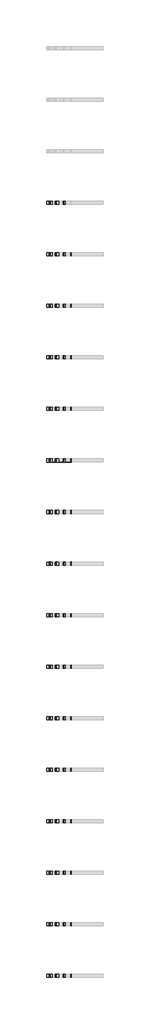
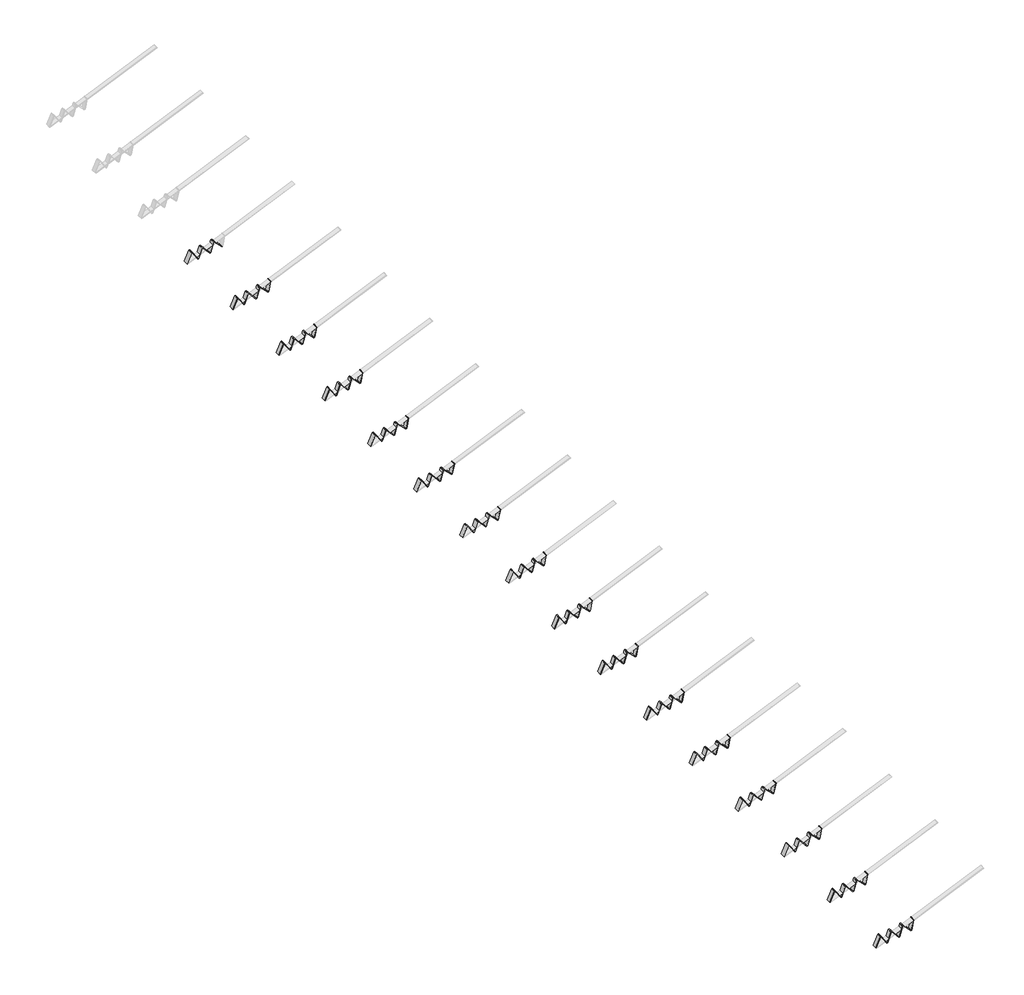
# One storey, part 1 of 4: 111 beams.
"""IFC4 building model written with IfcOpenShell, lengths in millimetres."""

import ifcopenshell
import ifcopenshell.guid

model = None  # the IFC model being written
_history = None  # IfcOwnerHistory: only IFC2X3 demands one
_inside = {}  # id of a spatial element -> (the spatial element, [elements in it])
_under = {}  # id of a project, library or spatial element -> (it, [spatial elements below it])
_declared = {}  # id of a project -> (the project, [libraries it declares])
_typed = {}  # id of a type object -> (the type object, [elements of that type])
_made_of = {}  # id of a material, layer set ... -> (it, [elements and type objects made of it])


def new_model(schema):
    """Start an empty IFC model of exactly this schema.

    Asked for "IFC4X3", IfcOpenShell would pick the latest addendum, in which some entities
    have other attributes; the version numbers below select the first issue.
    IFC2X3 requires an IfcOwnerHistory on every rooted entity: one is made here for all.
    """
    global model, _history
    if schema == "IFC4X3":
        model = ifcopenshell.file(schema_version=(4, 3, 0, 0))
    else:
        model = ifcopenshell.file(schema=schema)
    _inside.clear()
    _under.clear()
    _declared.clear()
    _typed.clear()
    _made_of.clear()
    _history = None
    if model.schema == "IFC2X3":
        org = make("IfcOrganization", Name="unknown")
        user = make(
            "IfcPersonAndOrganization",
            ThePerson=make("IfcPerson", FamilyName="unknown"),
            TheOrganization=org,
        )
        app = make(
            "IfcApplication",
            ApplicationDeveloper=org,
            Version="unknown",
            ApplicationFullName="unknown",
            ApplicationIdentifier="unknown",
        )
        _history = make(
            "IfcOwnerHistory",
            OwningUser=user,
            OwningApplication=app,
            ChangeAction="ADDED",
            CreationDate=0,
        )
    return model


def make(cls, **values):
    """One entity of the class cls with the attributes given. An attribute that is None is left unset."""
    return model.create_entity(
        cls, **{name: value for name, value in values.items() if value is not None}
    )


def rooted(cls, **values):
    """An entity with a GlobalId (a new one), such as an element, a storey or a relation."""
    return make(cls, GlobalId=ifcopenshell.guid.new(), OwnerHistory=_history, **values)


def si_unit(unit_type, name, prefix=None):
    """IfcSIUnit, for example si_unit("LENGTHUNIT", "METRE", prefix="MILLI")."""
    return make("IfcSIUnit", UnitType=unit_type, Prefix=prefix, Name=name)


def assignment(units):
    """IfcUnitAssignment: the units of a project."""
    return None if units is None else make("IfcUnitAssignment", Units=units)


def point(xyz):
    """IfcCartesianPoint."""
    return None if xyz is None else make("IfcCartesianPoint", Coordinates=xyz)


def direction(xyz):
    """IfcDirection."""
    return None if xyz is None else make("IfcDirection", DirectionRatios=xyz)


def frame(location, z_axis=None, x_axis=None):
    """IfcAxis2Placement3D, a coordinate frame: its origin and axes. An axis left out is left unset."""
    return make(
        "IfcAxis2Placement3D",
        Location=point(location),
        Axis=direction(z_axis),
        RefDirection=direction(x_axis),
    )


def origin():
    """The frame at (0, 0, 0) with its axes left unset."""
    return frame((0.0, 0.0, 0.0))


def place(relative_to, where):
    """IfcLocalPlacement: puts the frame where relative to a parent placement (None: the world)."""
    return make(
        "IfcLocalPlacement", PlacementRelTo=relative_to, RelativePlacement=where
    )


def context(
    kind, dimensions, precision=None, world=None, true_north=None, identifier=None
):
    """IfcGeometricRepresentationContext, for example the 3D "Model" context."""
    return make(
        "IfcGeometricRepresentationContext",
        ContextIdentifier=identifier,
        ContextType=kind,
        CoordinateSpaceDimension=dimensions,
        Precision=precision,
        WorldCoordinateSystem=world,
        TrueNorth=true_north,
    )


def project(units=None, contexts=None):
    """IfcProject with its units and contexts."""
    return rooted(
        "IfcProject",
        Name="project",
        RepresentationContexts=contexts,
        UnitsInContext=assignment(units),
    )


def spatial(cls, under=None, at=None, **own):
    """A site, building, storey or space (cls), placed at a placement, below another one or the project."""
    s = rooted(cls, ObjectPlacement=at, **own)
    if under is not None:
        _under.setdefault(under.id(), (under, []))[1].append(s)
    return s


def polyline(points):
    """IfcPolyline through the points."""
    return make("IfcPolyline", Points=[point(p) for p in points])


def outline(outer, holes=None, kind="AREA"):
    """IfcArbitraryClosedProfileDef: a profile drawn as a closed curve; with holes, ...WithVoids."""
    if holes is None:
        return make("IfcArbitraryClosedProfileDef", ProfileType=kind, OuterCurve=outer)
    return make(
        "IfcArbitraryProfileDefWithVoids",
        ProfileType=kind,
        OuterCurve=outer,
        InnerCurves=holes,
    )


def extrude(swept, where, along, depth):
    """IfcExtrudedAreaSolid: the profile swept, set in the frame where, extruded along a direction by depth."""
    return make(
        "IfcExtrudedAreaSolid",
        SweptArea=swept,
        Position=where,
        ExtrudedDirection=direction(along),
        Depth=depth,
    )


def shape(context_of_items, identifier, shape_type, items):
    """IfcShapeRepresentation: the items that make up one representation, for example the "Body"."""
    return make(
        "IfcShapeRepresentation",
        ContextOfItems=context_of_items,
        RepresentationIdentifier=identifier,
        RepresentationType=shape_type,
        Items=items,
    )


def source(mapping_origin, context_of_items, identifier, shape_type, items):
    """IfcRepresentationMap: a shape defined once, which mapped items show again and again."""
    return make(
        "IfcRepresentationMap",
        MappingOrigin=mapping_origin,
        MappedRepresentation=shape(context_of_items, identifier, shape_type, items),
    )


def transform(
    local_origin,
    x_axis=None,
    y_axis=None,
    z_axis=None,
    scale=None,
    scale2=None,
    scale3=None,
    uniform=True,
):
    """IfcCartesianTransformationOperator3D, or its non-uniform kind. x_axis, y_axis, z_axis: its Axis1, 2, 3."""
    if uniform:
        return make(
            "IfcCartesianTransformationOperator3D",
            Axis1=direction(x_axis),
            Axis2=direction(y_axis),
            LocalOrigin=point(local_origin),
            Scale=scale,
            Axis3=direction(z_axis),
        )
    return make(
        "IfcCartesianTransformationOperator3DnonUniform",
        Axis1=direction(x_axis),
        Axis2=direction(y_axis),
        LocalOrigin=point(local_origin),
        Scale=scale,
        Axis3=direction(z_axis),
        Scale2=scale2,
        Scale3=scale3,
    )


def mapped(mapping_source, mapping_target):
    """IfcMappedItem: shows the shape of a source again, moved by a transform."""
    return make(
        "IfcMappedItem", MappingSource=mapping_source, MappingTarget=mapping_target
    )


def made_of(thing, what):
    """Note that an element or type object is made of a material, layer set ...; save() writes the relation."""
    if what is not None:
        _made_of.setdefault(what.id(), (what, []))[1].append(thing)
    return thing


def element(
    cls,
    number,
    at=None,
    inside=None,
    cuts=None,
    type_object=None,
    material=None,
    context=None,
    identifier="Body",
    shape_type=None,
    held_by="IfcProductDefinitionShape",
    body=None,
    shapes=None,
    **own,
):
    """One element of the class cls, such as IfcWall. Its Tag is "e" and its number.

    at: its placement. inside: the storey or other place that contains it. cuts: it is an
    opening in that element (IfcRelVoidsElement). A single representation is given by context,
    identifier, shape_type and body (its items); several are given by shapes. held_by: the class
    of the entity that holds the representations. save() writes the other relations.
    """
    e = rooted(cls, Tag="e%d" % number, ObjectPlacement=at, **own)
    if body is not None:
        shapes = [shape(context, identifier, shape_type, body)]
    if shapes is not None:
        e.Representation = make(held_by, Representations=shapes)
    if inside is not None:
        _inside.setdefault(inside.id(), (inside, []))[1].append(e)
    if cuts is not None:
        rooted(
            "IfcRelVoidsElement", RelatingBuildingElement=cuts, RelatedOpeningElement=e
        )
    if type_object is not None:
        _typed.setdefault(type_object.id(), (type_object, []))[1].append(e)
    return made_of(e, material)


def aggregate(whole, parts):
    """IfcRelAggregates: a whole, such as a stair, and the parts it consists of."""
    return rooted("IfcRelAggregates", RelatingObject=whole, RelatedObjects=parts)


def save(model, path):
    """Write the relations noted so far, then the file.

    IfcRelAggregates (storeys below a building ...), IfcRelContainedInSpatialStructure (elements
    in a storey), IfcRelDefinesByType, IfcRelAssociatesMaterial and IfcRelDeclares: one each for
    every whole, place, type object, material and project.
    """
    for whole, parts in _under.values():
        aggregate(whole, parts)
    for where, things in _inside.values():
        rooted(
            "IfcRelContainedInSpatialStructure",
            RelatedElements=things,
            RelatingStructure=where,
        )
    for kind, things in _typed.values():
        rooted("IfcRelDefinesByType", RelatedObjects=things, RelatingType=kind)
    for what, things in _made_of.values():
        rooted("IfcRelAssociatesMaterial", RelatedObjects=things, RelatingMaterial=what)
    for by, libraries in _declared.values():
        rooted("IfcRelDeclares", RelatingContext=by, RelatedDefinitions=libraries)
    model.write(path)


def placa_diagonal_a71479e9(model_context):
    return source(origin(), model_context, "Body", "SweptSolid", [
        extrude(outline(polyline([(161.178496, 75.0), (161.178496, -75.0), (-185.3041805, -75.0), (-185.3041805, 75.0), (161.178496, 75.0)])), frame((0.0, 0.0, -4.0), z_axis=(0.0, 0.0, 1.0), x_axis=(1.0, 0.0, 0.0)), (0.0, 0.0, 1.0), 8.0),
    ])


def placa_diagonal_67ce8334(model_context):
    return source(origin(), model_context, "Body", "SweptSolid", [
        extrude(outline(polyline([(162.9623469, 75.0), (162.9623469, -75.0), (-162.6761246, -75.0), (-162.6761246, 75.0), (162.9623469, 75.0)])), frame((0.0, 0.0, -4.0), z_axis=(0.0, 0.0, 1.0), x_axis=(1.0, 0.0, 0.0)), (0.0, 0.0, 1.0), 8.0),
    ])


def placa_diagonal_af2a04a3(model_context):
    return source(origin(), model_context, "Body", "SweptSolid", [
        extrude(outline(polyline([(165.1705216, 75.0), (165.1705216, -75.0), (-165.4962729, -75.0), (-165.4962729, 75.0), (165.1705216, 75.0)])), frame((0.0, 0.0, -4.0), z_axis=(0.0, 0.0, 1.0), x_axis=(1.0, 0.0, 0.0)), (0.0, 0.0, 1.0), 8.0),
    ])


def placa_diagonal_fb53ba7d(model_context):
    return source(origin(), model_context, "Body", "SweptSolid", [
        extrude(outline(polyline([(169.971959, 75.0), (169.971959, -75.0), (-169.5739242, -75.0), (-169.5739242, 75.0), (169.971959, 75.0)])), frame((0.0, 0.0, -4.0), z_axis=(0.0, 0.0, 1.0), x_axis=(1.0, 0.0, 0.0)), (0.0, 0.0, 1.0), 8.0),
    ])


def placa_diagonal_d1da0e1c(model_context):
    return source(origin(), model_context, "Body", "SweptSolid", [
        extrude(outline(polyline([(165.1705221, 75.0), (165.1705221, -75.0), (-165.4962734, -75.0), (-165.4962734, 75.0), (165.1705221, 75.0)])), frame((0.0, 0.0, -4.0), z_axis=(0.0, 0.0, 1.0), x_axis=(1.0, 0.0, 0.0)), (0.0, 0.0, 1.0), 8.0),
    ])


model = new_model("IFC4")

# Units and contexts
model_context = context("Model", 3, world=origin())
ifc_project = project(units=[si_unit("LENGTHUNIT", "METRE", prefix="MILLI")], contexts=[model_context])

# Site, building, storey
site = spatial("IfcSite", under=ifc_project)
building = spatial("IfcBuilding", under=site)
storey = spatial("IfcBuildingStorey", under=building, Name="Nível 4", Elevation=48165.0)

# Beams
placement = place(None, origin())
placa_diagonal_shape = placa_diagonal_a71479e9(model_context)
element("IfcBeam", 1, ObjectType="Placa : diagonal", at=placement, inside=storey, context=model_context, shape_type="MappedRepresentation", body=[
    mapped(placa_diagonal_shape, transform((-1468.5029422, -39603.5623634, 48342.5238752), x_axis=(0.4074605623535313, 0.0, 0.9132228042085588), y_axis=(0.0, -1.0, 0.0), z_axis=(0.9132228042085588, 0.0, -0.4074605623535313))),
])
element("IfcBeam", 2, ObjectType="Placa : diagonal", at=placement, inside=storey, context=model_context, shape_type="MappedRepresentation", body=[
    mapped(placa_diagonal_shape, transform((-1468.5029422, -2103.5623634, 48342.5238752), x_axis=(0.4074605623535313, 0.0, 0.9132228042085588), y_axis=(0.0, -1.0, 0.0), z_axis=(0.9132228042085588, 0.0, -0.4074605623535313))),
])
element("IfcBeam", 3, ObjectType="Placa : diagonal", at=placement, inside=storey, context=model_context, shape_type="MappedRepresentation", body=[
    mapped(placa_diagonal_shape, transform((-1468.5029422, -4603.5623634, 48342.5238752), x_axis=(0.4074605623535313, 0.0, 0.9132228042085588), y_axis=(0.0, -1.0, 0.0), z_axis=(0.9132228042085588, 0.0, -0.4074605623535313))),
])
element("IfcBeam", 4, ObjectType="Placa : diagonal", at=placement, inside=storey, context=model_context, shape_type="MappedRepresentation", body=[
    mapped(placa_diagonal_shape, transform((-1468.5029422, -7103.5623634, 48342.5238752), x_axis=(0.4074605623535313, 0.0, 0.9132228042085588), y_axis=(0.0, -1.0, 0.0), z_axis=(0.9132228042085588, 0.0, -0.4074605623535313))),
])
element("IfcBeam", 5, ObjectType="Placa : diagonal", at=placement, inside=storey, context=model_context, shape_type="MappedRepresentation", body=[
    mapped(placa_diagonal_shape, transform((-1468.5029422, -9603.5623634, 48342.5238752), x_axis=(0.4074605623535313, 0.0, 0.9132228042085588), y_axis=(0.0, -1.0, 0.0), z_axis=(0.9132228042085588, 0.0, -0.4074605623535313))),
])
element("IfcBeam", 6, ObjectType="Placa : diagonal", at=placement, inside=storey, context=model_context, shape_type="MappedRepresentation", body=[
    mapped(placa_diagonal_shape, transform((-1468.5029422, -12103.5623634, 48342.5238752), x_axis=(0.4074605623535313, 0.0, 0.9132228042085588), y_axis=(0.0, -1.0, 0.0), z_axis=(0.9132228042085588, 0.0, -0.4074605623535313))),
])
element("IfcBeam", 7, ObjectType="Placa : diagonal", at=placement, inside=storey, context=model_context, shape_type="MappedRepresentation", body=[
    mapped(placa_diagonal_shape, transform((-1468.5029422, -14603.5623634, 48342.5238752), x_axis=(0.4074605623535313, 0.0, 0.9132228042085588), y_axis=(0.0, -1.0, 0.0), z_axis=(0.9132228042085588, 0.0, -0.4074605623535313))),
])
element("IfcBeam", 8, ObjectType="Placa : diagonal", at=placement, inside=storey, context=model_context, shape_type="MappedRepresentation", body=[
    mapped(placa_diagonal_shape, transform((-1468.5029422, -17103.5623634, 48342.5238752), x_axis=(0.4074605623535313, 0.0, 0.9132228042085588), y_axis=(0.0, -1.0, 0.0), z_axis=(0.9132228042085588, 0.0, -0.4074605623535313))),
])
element("IfcBeam", 9, ObjectType="Placa : diagonal", at=placement, inside=storey, context=model_context, shape_type="MappedRepresentation", body=[
    mapped(placa_diagonal_shape, transform((-1468.5029422, -19603.5623634, 48342.5238752), x_axis=(0.4074605623535313, 0.0, 0.9132228042085588), y_axis=(0.0, -1.0, 0.0), z_axis=(0.9132228042085588, 0.0, -0.4074605623535313))),
])
element("IfcBeam", 10, ObjectType="Placa : diagonal", at=placement, inside=storey, context=model_context, shape_type="MappedRepresentation", body=[
    mapped(placa_diagonal_shape, transform((-1468.5029422, -22103.5623634, 48342.5238752), x_axis=(0.4074605623535313, 0.0, 0.9132228042085588), y_axis=(0.0, -1.0, 0.0), z_axis=(0.9132228042085588, 0.0, -0.4074605623535313))),
])
element("IfcBeam", 11, ObjectType="Placa : diagonal", at=placement, inside=storey, context=model_context, shape_type="MappedRepresentation", body=[
    mapped(placa_diagonal_shape, transform((-1468.5029422, -24603.5623634, 48342.5238752), x_axis=(0.4074605623535313, 0.0, 0.9132228042085588), y_axis=(0.0, -1.0, 0.0), z_axis=(0.9132228042085588, 0.0, -0.4074605623535313))),
])
element("IfcBeam", 12, ObjectType="Placa : diagonal", at=placement, inside=storey, context=model_context, shape_type="MappedRepresentation", body=[
    mapped(placa_diagonal_shape, transform((-1468.5029422, -27103.5623634, 48342.5238752), x_axis=(0.4074605623535313, 0.0, 0.9132228042085588), y_axis=(0.0, -1.0, 0.0), z_axis=(0.9132228042085588, 0.0, -0.4074605623535313))),
])
element("IfcBeam", 13, ObjectType="Placa : diagonal", at=placement, inside=storey, context=model_context, shape_type="MappedRepresentation", body=[
    mapped(placa_diagonal_shape, transform((-1468.5029422, -29603.5623634, 48342.5238752), x_axis=(0.4074605623535313, 0.0, 0.9132228042085588), y_axis=(0.0, -1.0, 0.0), z_axis=(0.9132228042085588, 0.0, -0.4074605623535313))),
])
element("IfcBeam", 14, ObjectType="Placa : diagonal", at=placement, inside=storey, context=model_context, shape_type="MappedRepresentation", body=[
    mapped(placa_diagonal_shape, transform((-1468.5029422, -32103.5623634, 48342.5238752), x_axis=(0.4074605623535313, 0.0, 0.9132228042085588), y_axis=(0.0, -1.0, 0.0), z_axis=(0.9132228042085588, 0.0, -0.4074605623535313))),
])
element("IfcBeam", 15, ObjectType="Placa : diagonal", at=placement, inside=storey, context=model_context, shape_type="MappedRepresentation", body=[
    mapped(placa_diagonal_shape, transform((-1468.5029422, -34603.5623634, 48342.5238752), x_axis=(0.4074605623535313, 0.0, 0.9132228042085588), y_axis=(0.0, -1.0, 0.0), z_axis=(0.9132228042085588, 0.0, -0.4074605623535313))),
])
element("IfcBeam", 16, ObjectType="Placa : diagonal", at=placement, inside=storey, context=model_context, shape_type="MappedRepresentation", body=[
    mapped(placa_diagonal_shape, transform((-1468.5029422, -37103.5623634, 48342.5238752), x_axis=(0.4074605623535313, 0.0, 0.9132228042085588), y_axis=(0.0, -1.0, 0.0), z_axis=(0.9132228042085588, 0.0, -0.4074605623535313))),
])
placa_diagonal_2_shape = placa_diagonal_67ce8334(model_context)
element("IfcBeam", 17, ObjectType="Placa : diagonal", at=placement, inside=storey, context=model_context, shape_type="MappedRepresentation", body=[
    mapped(placa_diagonal_2_shape, transform((-1292.3410904, -39603.5623634, 48354.815057), x_axis=(0.5398932132172984, 0.0, -0.8417335197803998), y_axis=(0.0, -1.0, 0.0), z_axis=(-0.8417335197803998, 0.0, -0.5398932132172984))),
])
element("IfcBeam", 18, ObjectType="Placa : diagonal", at=placement, inside=storey, context=model_context, shape_type="MappedRepresentation", body=[
    mapped(placa_diagonal_2_shape, transform((-1292.3410904, -2103.5623634, 48354.815057), x_axis=(0.5398932132172984, 0.0, -0.8417335197803998), y_axis=(0.0, -1.0, 0.0), z_axis=(-0.8417335197803998, 0.0, -0.5398932132172984))),
])
element("IfcBeam", 19, ObjectType="Placa : diagonal", at=placement, inside=storey, context=model_context, shape_type="MappedRepresentation", body=[
    mapped(placa_diagonal_2_shape, transform((-1292.3410904, -4603.5623634, 48354.815057), x_axis=(0.5398932132172984, 0.0, -0.8417335197803998), y_axis=(0.0, -1.0, 0.0), z_axis=(-0.8417335197803998, 0.0, -0.5398932132172984))),
])
element("IfcBeam", 20, ObjectType="Placa : diagonal", at=placement, inside=storey, context=model_context, shape_type="MappedRepresentation", body=[
    mapped(placa_diagonal_2_shape, transform((-1292.3410904, -7103.5623634, 48354.815057), x_axis=(0.5398932132172984, 0.0, -0.8417335197803998), y_axis=(0.0, -1.0, 0.0), z_axis=(-0.8417335197803998, 0.0, -0.5398932132172984))),
])
element("IfcBeam", 21, ObjectType="Placa : diagonal", at=placement, inside=storey, context=model_context, shape_type="MappedRepresentation", body=[
    mapped(placa_diagonal_2_shape, transform((-1292.3410904, -9603.5623634, 48354.815057), x_axis=(0.5398932132172984, 0.0, -0.8417335197803998), y_axis=(0.0, -1.0, 0.0), z_axis=(-0.8417335197803998, 0.0, -0.5398932132172984))),
])
element("IfcBeam", 22, ObjectType="Placa : diagonal", at=placement, inside=storey, context=model_context, shape_type="MappedRepresentation", body=[
    mapped(placa_diagonal_2_shape, transform((-1292.3410904, -12103.5623634, 48354.815057), x_axis=(0.5398932132172984, 0.0, -0.8417335197803998), y_axis=(0.0, -1.0, 0.0), z_axis=(-0.8417335197803998, 0.0, -0.5398932132172984))),
])
element("IfcBeam", 23, ObjectType="Placa : diagonal", at=placement, inside=storey, context=model_context, shape_type="MappedRepresentation", body=[
    mapped(placa_diagonal_2_shape, transform((-1292.3410904, -14603.5623634, 48354.815057), x_axis=(0.5398932132172984, 0.0, -0.8417335197803998), y_axis=(0.0, -1.0, 0.0), z_axis=(-0.8417335197803998, 0.0, -0.5398932132172984))),
])
element("IfcBeam", 24, ObjectType="Placa : diagonal", at=placement, inside=storey, context=model_context, shape_type="MappedRepresentation", body=[
    mapped(placa_diagonal_2_shape, transform((-1292.3410904, -17103.5623634, 48354.815057), x_axis=(0.5398932132172984, 0.0, -0.8417335197803998), y_axis=(0.0, -1.0, 0.0), z_axis=(-0.8417335197803998, 0.0, -0.5398932132172984))),
])
element("IfcBeam", 25, ObjectType="Placa : diagonal", at=placement, inside=storey, context=model_context, shape_type="MappedRepresentation", body=[
    mapped(placa_diagonal_2_shape, transform((-1292.3410904, -19603.5623634, 48354.815057), x_axis=(0.5398932132172984, 0.0, -0.8417335197803998), y_axis=(0.0, -1.0, 0.0), z_axis=(-0.8417335197803998, 0.0, -0.5398932132172984))),
])
element("IfcBeam", 26, ObjectType="Placa : diagonal", at=placement, inside=storey, context=model_context, shape_type="MappedRepresentation", body=[
    mapped(placa_diagonal_2_shape, transform((-1292.3410904, -22103.5623634, 48354.815057), x_axis=(0.5398932132172984, 0.0, -0.8417335197803998), y_axis=(0.0, -1.0, 0.0), z_axis=(-0.8417335197803998, 0.0, -0.5398932132172984))),
])
element("IfcBeam", 27, ObjectType="Placa : diagonal", at=placement, inside=storey, context=model_context, shape_type="MappedRepresentation", body=[
    mapped(placa_diagonal_2_shape, transform((-1292.3410904, -24603.5623634, 48354.815057), x_axis=(0.5398932132172984, 0.0, -0.8417335197803998), y_axis=(0.0, -1.0, 0.0), z_axis=(-0.8417335197803998, 0.0, -0.5398932132172984))),
])
element("IfcBeam", 28, ObjectType="Placa : diagonal", at=placement, inside=storey, context=model_context, shape_type="MappedRepresentation", body=[
    mapped(placa_diagonal_2_shape, transform((-1292.3410904, -27103.5623634, 48354.815057), x_axis=(0.5398932132172984, 0.0, -0.8417335197803998), y_axis=(0.0, -1.0, 0.0), z_axis=(-0.8417335197803998, 0.0, -0.5398932132172984))),
])
element("IfcBeam", 29, ObjectType="Placa : diagonal", at=placement, inside=storey, context=model_context, shape_type="MappedRepresentation", body=[
    mapped(placa_diagonal_2_shape, transform((-1292.3410904, -29603.5623634, 48354.815057), x_axis=(0.5398932132172984, 0.0, -0.8417335197803998), y_axis=(0.0, -1.0, 0.0), z_axis=(-0.8417335197803998, 0.0, -0.5398932132172984))),
])
element("IfcBeam", 30, ObjectType="Placa : diagonal", at=placement, inside=storey, context=model_context, shape_type="MappedRepresentation", body=[
    mapped(placa_diagonal_2_shape, transform((-1292.3410904, -32103.5623634, 48354.815057), x_axis=(0.5398932132172984, 0.0, -0.8417335197803998), y_axis=(0.0, -1.0, 0.0), z_axis=(-0.8417335197803998, 0.0, -0.5398932132172984))),
])
element("IfcBeam", 31, ObjectType="Placa : diagonal", at=placement, inside=storey, context=model_context, shape_type="MappedRepresentation", body=[
    mapped(placa_diagonal_2_shape, transform((-1292.3410904, -34603.5623634, 48354.815057), x_axis=(0.5398932132172984, 0.0, -0.8417335197803998), y_axis=(0.0, -1.0, 0.0), z_axis=(-0.8417335197803998, 0.0, -0.5398932132172984))),
])
element("IfcBeam", 32, ObjectType="Placa : diagonal", at=placement, inside=storey, context=model_context, shape_type="MappedRepresentation", body=[
    mapped(placa_diagonal_2_shape, transform((-1292.3410904, -37103.5623634, 48354.815057), x_axis=(0.5398932132172984, 0.0, -0.8417335197803998), y_axis=(0.0, -1.0, 0.0), z_axis=(-0.8417335197803998, 0.0, -0.5398932132172984))),
])
placa_diagonal_3_shape = placa_diagonal_af2a04a3(model_context)
element("IfcBeam", 33, ObjectType="Placa : diagonal", at=placement, inside=storey, context=model_context, shape_type="MappedRepresentation", body=[
    mapped(placa_diagonal_3_shape, transform((-1127.2550828, -39603.5623634, 48375.8118772), x_axis=(0.3404667803509138, 0.0, 0.940256545564817), y_axis=(0.0, -1.0, 0.0), z_axis=(0.940256545564817, 0.0, -0.3404667803509138))),
])
element("IfcBeam", 34, ObjectType="Placa : diagonal", at=placement, inside=storey, context=model_context, shape_type="MappedRepresentation", body=[
    mapped(placa_diagonal_3_shape, transform((-392.7303205, -39603.5623634, 48535.8666224), x_axis=(0.20085127706480188, 0.0, 0.9796217456250337), y_axis=(0.0, -1.0, 0.0), z_axis=(0.9796217456250337, 0.0, -0.20085127706480188))),
])
element("IfcBeam", 35, ObjectType="Placa : diagonal", at=placement, inside=storey, context=model_context, shape_type="MappedRepresentation", body=[
    mapped(placa_diagonal_3_shape, transform((-1127.2550828, -2103.5623634, 48375.8118772), x_axis=(0.3404667803509138, 0.0, 0.940256545564817), y_axis=(0.0, -1.0, 0.0), z_axis=(0.940256545564817, 0.0, -0.3404667803509138))),
])
element("IfcBeam", 36, ObjectType="Placa : diagonal", at=placement, inside=storey, context=model_context, shape_type="MappedRepresentation", body=[
    mapped(placa_diagonal_3_shape, transform((-1127.2550828, -4603.5623634, 48375.8118772), x_axis=(0.3404667803509138, 0.0, 0.940256545564817), y_axis=(0.0, -1.0, 0.0), z_axis=(0.940256545564817, 0.0, -0.3404667803509138))),
])
element("IfcBeam", 37, ObjectType="Placa : diagonal", at=placement, inside=storey, context=model_context, shape_type="MappedRepresentation", body=[
    mapped(placa_diagonal_3_shape, transform((-392.7303205, -4603.5623634, 48535.8666224), x_axis=(0.20085127706480188, 0.0, 0.9796217456250337), y_axis=(0.0, -1.0, 0.0), z_axis=(0.9796217456250337, 0.0, -0.20085127706480188))),
])
element("IfcBeam", 38, ObjectType="Placa : diagonal", at=placement, inside=storey, context=model_context, shape_type="MappedRepresentation", body=[
    mapped(placa_diagonal_3_shape, transform((-1127.2550828, -7103.5623634, 48375.8118772), x_axis=(0.3404667803509138, 0.0, 0.940256545564817), y_axis=(0.0, -1.0, 0.0), z_axis=(0.940256545564817, 0.0, -0.3404667803509138))),
])
element("IfcBeam", 39, ObjectType="Placa : diagonal", at=placement, inside=storey, context=model_context, shape_type="MappedRepresentation", body=[
    mapped(placa_diagonal_3_shape, transform((-392.7303205, -7103.5623634, 48535.8666224), x_axis=(0.20085127706480188, 0.0, 0.9796217456250337), y_axis=(0.0, -1.0, 0.0), z_axis=(0.9796217456250337, 0.0, -0.20085127706480188))),
])
element("IfcBeam", 40, ObjectType="Placa : diagonal", at=placement, inside=storey, context=model_context, shape_type="MappedRepresentation", body=[
    mapped(placa_diagonal_3_shape, transform((-1127.2550828, -9603.5623634, 48375.8118772), x_axis=(0.3404667803509138, 0.0, 0.940256545564817), y_axis=(0.0, -1.0, 0.0), z_axis=(0.940256545564817, 0.0, -0.3404667803509138))),
])
element("IfcBeam", 41, ObjectType="Placa : diagonal", at=placement, inside=storey, context=model_context, shape_type="MappedRepresentation", body=[
    mapped(placa_diagonal_3_shape, transform((-392.7303205, -9603.5623634, 48535.8666224), x_axis=(0.20085127706480188, 0.0, 0.9796217456250337), y_axis=(0.0, -1.0, 0.0), z_axis=(0.9796217456250337, 0.0, -0.20085127706480188))),
])
element("IfcBeam", 42, ObjectType="Placa : diagonal", at=placement, inside=storey, context=model_context, shape_type="MappedRepresentation", body=[
    mapped(placa_diagonal_3_shape, transform((-1127.2550828, -12103.5623634, 48375.8118772), x_axis=(0.3404667803509138, 0.0, 0.940256545564817), y_axis=(0.0, -1.0, 0.0), z_axis=(0.940256545564817, 0.0, -0.3404667803509138))),
])
element("IfcBeam", 43, ObjectType="Placa : diagonal", at=placement, inside=storey, context=model_context, shape_type="MappedRepresentation", body=[
    mapped(placa_diagonal_3_shape, transform((-392.7303205, -12103.5623634, 48535.8666224), x_axis=(0.20085127706480188, 0.0, 0.9796217456250337), y_axis=(0.0, -1.0, 0.0), z_axis=(0.9796217456250337, 0.0, -0.20085127706480188))),
])
element("IfcBeam", 44, ObjectType="Placa : diagonal", at=placement, inside=storey, context=model_context, shape_type="MappedRepresentation", body=[
    mapped(placa_diagonal_3_shape, transform((-1127.2550828, -14603.5623634, 48375.8118772), x_axis=(0.3404667803509138, 0.0, 0.940256545564817), y_axis=(0.0, -1.0, 0.0), z_axis=(0.940256545564817, 0.0, -0.3404667803509138))),
])
element("IfcBeam", 45, ObjectType="Placa : diagonal", at=placement, inside=storey, context=model_context, shape_type="MappedRepresentation", body=[
    mapped(placa_diagonal_3_shape, transform((-392.7303205, -14603.5623634, 48535.8666224), x_axis=(0.20085127706480188, 0.0, 0.9796217456250337), y_axis=(0.0, -1.0, 0.0), z_axis=(0.9796217456250337, 0.0, -0.20085127706480188))),
])
element("IfcBeam", 46, ObjectType="Placa : diagonal", at=placement, inside=storey, context=model_context, shape_type="MappedRepresentation", body=[
    mapped(placa_diagonal_3_shape, transform((-1127.2550828, -17103.5623634, 48375.8118772), x_axis=(0.3404667803509138, 0.0, 0.940256545564817), y_axis=(0.0, -1.0, 0.0), z_axis=(0.940256545564817, 0.0, -0.3404667803509138))),
])
element("IfcBeam", 47, ObjectType="Placa : diagonal", at=placement, inside=storey, context=model_context, shape_type="MappedRepresentation", body=[
    mapped(placa_diagonal_3_shape, transform((-392.7303205, -17103.5623634, 48535.8666224), x_axis=(0.20085127706480188, 0.0, 0.9796217456250337), y_axis=(0.0, -1.0, 0.0), z_axis=(0.9796217456250337, 0.0, -0.20085127706480188))),
])
element("IfcBeam", 48, ObjectType="Placa : diagonal", at=placement, inside=storey, context=model_context, shape_type="MappedRepresentation", body=[
    mapped(placa_diagonal_3_shape, transform((-1127.2550828, -19603.5623634, 48375.8118772), x_axis=(0.3404667803509138, 0.0, 0.940256545564817), y_axis=(0.0, -1.0, 0.0), z_axis=(0.940256545564817, 0.0, -0.3404667803509138))),
])
element("IfcBeam", 49, ObjectType="Placa : diagonal", at=placement, inside=storey, context=model_context, shape_type="MappedRepresentation", body=[
    mapped(placa_diagonal_3_shape, transform((-392.7303205, -19603.5623634, 48535.8666224), x_axis=(0.20085127706480188, 0.0, 0.9796217456250337), y_axis=(0.0, -1.0, 0.0), z_axis=(0.9796217456250337, 0.0, -0.20085127706480188))),
])
element("IfcBeam", 50, ObjectType="Placa : diagonal", at=placement, inside=storey, context=model_context, shape_type="MappedRepresentation", body=[
    mapped(placa_diagonal_3_shape, transform((-1127.2550828, -22103.5623634, 48375.8118772), x_axis=(0.3404667803509138, 0.0, 0.940256545564817), y_axis=(0.0, -1.0, 0.0), z_axis=(0.940256545564817, 0.0, -0.3404667803509138))),
])
element("IfcBeam", 51, ObjectType="Placa : diagonal", at=placement, inside=storey, context=model_context, shape_type="MappedRepresentation", body=[
    mapped(placa_diagonal_3_shape, transform((-392.7303205, -22103.5623634, 48535.8666224), x_axis=(0.20085127706480188, 0.0, 0.9796217456250337), y_axis=(0.0, -1.0, 0.0), z_axis=(0.9796217456250337, 0.0, -0.20085127706480188))),
])
element("IfcBeam", 52, ObjectType="Placa : diagonal", at=placement, inside=storey, context=model_context, shape_type="MappedRepresentation", body=[
    mapped(placa_diagonal_3_shape, transform((-1127.2550828, -24603.5623634, 48375.8118772), x_axis=(0.3404667803509138, 0.0, 0.940256545564817), y_axis=(0.0, -1.0, 0.0), z_axis=(0.940256545564817, 0.0, -0.3404667803509138))),
])
element("IfcBeam", 53, ObjectType="Placa : diagonal", at=placement, inside=storey, context=model_context, shape_type="MappedRepresentation", body=[
    mapped(placa_diagonal_3_shape, transform((-392.7303205, -24603.5623634, 48535.8666224), x_axis=(0.20085127706480188, 0.0, 0.9796217456250337), y_axis=(0.0, -1.0, 0.0), z_axis=(0.9796217456250337, 0.0, -0.20085127706480188))),
])
element("IfcBeam", 54, ObjectType="Placa : diagonal", at=placement, inside=storey, context=model_context, shape_type="MappedRepresentation", body=[
    mapped(placa_diagonal_3_shape, transform((-1127.2550828, -27103.5623634, 48375.8118772), x_axis=(0.3404667803509138, 0.0, 0.940256545564817), y_axis=(0.0, -1.0, 0.0), z_axis=(0.940256545564817, 0.0, -0.3404667803509138))),
])
element("IfcBeam", 55, ObjectType="Placa : diagonal", at=placement, inside=storey, context=model_context, shape_type="MappedRepresentation", body=[
    mapped(placa_diagonal_3_shape, transform((-392.7303205, -27103.5623634, 48535.8666224), x_axis=(0.20085127706480188, 0.0, 0.9796217456250337), y_axis=(0.0, -1.0, 0.0), z_axis=(0.9796217456250337, 0.0, -0.20085127706480188))),
])
element("IfcBeam", 56, ObjectType="Placa : diagonal", at=placement, inside=storey, context=model_context, shape_type="MappedRepresentation", body=[
    mapped(placa_diagonal_3_shape, transform((-1127.2550828, -29603.5623634, 48375.8118772), x_axis=(0.3404667803509138, 0.0, 0.940256545564817), y_axis=(0.0, -1.0, 0.0), z_axis=(0.940256545564817, 0.0, -0.3404667803509138))),
])
element("IfcBeam", 57, ObjectType="Placa : diagonal", at=placement, inside=storey, context=model_context, shape_type="MappedRepresentation", body=[
    mapped(placa_diagonal_3_shape, transform((-392.7303205, -29603.5623634, 48535.8666224), x_axis=(0.20085127706480188, 0.0, 0.9796217456250337), y_axis=(0.0, -1.0, 0.0), z_axis=(0.9796217456250337, 0.0, -0.20085127706480188))),
])
element("IfcBeam", 58, ObjectType="Placa : diagonal", at=placement, inside=storey, context=model_context, shape_type="MappedRepresentation", body=[
    mapped(placa_diagonal_3_shape, transform((-1127.2550828, -32103.5623634, 48375.8118772), x_axis=(0.3404667803509138, 0.0, 0.940256545564817), y_axis=(0.0, -1.0, 0.0), z_axis=(0.940256545564817, 0.0, -0.3404667803509138))),
])
element("IfcBeam", 59, ObjectType="Placa : diagonal", at=placement, inside=storey, context=model_context, shape_type="MappedRepresentation", body=[
    mapped(placa_diagonal_3_shape, transform((-392.7303205, -32103.5623634, 48535.8666224), x_axis=(0.20085127706480188, 0.0, 0.9796217456250337), y_axis=(0.0, -1.0, 0.0), z_axis=(0.9796217456250337, 0.0, -0.20085127706480188))),
])
element("IfcBeam", 60, ObjectType="Placa : diagonal", at=placement, inside=storey, context=model_context, shape_type="MappedRepresentation", body=[
    mapped(placa_diagonal_3_shape, transform((-1127.2550828, -34603.5623634, 48375.8118772), x_axis=(0.3404667803509138, 0.0, 0.940256545564817), y_axis=(0.0, -1.0, 0.0), z_axis=(0.940256545564817, 0.0, -0.3404667803509138))),
])
element("IfcBeam", 61, ObjectType="Placa : diagonal", at=placement, inside=storey, context=model_context, shape_type="MappedRepresentation", body=[
    mapped(placa_diagonal_3_shape, transform((-392.7303205, -34603.5623634, 48535.8666224), x_axis=(0.20085127706480188, 0.0, 0.9796217456250337), y_axis=(0.0, -1.0, 0.0), z_axis=(0.9796217456250337, 0.0, -0.20085127706480188))),
])
element("IfcBeam", 62, ObjectType="Placa : diagonal", at=placement, inside=storey, context=model_context, shape_type="MappedRepresentation", body=[
    mapped(placa_diagonal_3_shape, transform((-1127.2550828, -37103.5623634, 48375.8118772), x_axis=(0.3404667803509138, 0.0, 0.940256545564817), y_axis=(0.0, -1.0, 0.0), z_axis=(0.940256545564817, 0.0, -0.3404667803509138))),
])
element("IfcBeam", 63, ObjectType="Placa : diagonal", at=placement, inside=storey, context=model_context, shape_type="MappedRepresentation", body=[
    mapped(placa_diagonal_3_shape, transform((-392.7303205, -37103.5623634, 48535.8666224), x_axis=(0.20085127706480188, 0.0, 0.9796217456250337), y_axis=(0.0, -1.0, 0.0), z_axis=(0.9796217456250337, 0.0, -0.20085127706480188))),
])
placa_diagonal_4_shape = placa_diagonal_fb53ba7d(model_context)
element("IfcBeam", 64, ObjectType="Placa : diagonal", at=placement, inside=storey, context=model_context, shape_type="MappedRepresentation", body=[
    mapped(placa_diagonal_4_shape, transform((-935.6334765, -39603.5623634, 48407.0552778), x_axis=(0.6551223780870831, 0.0, -0.7555227790937377), y_axis=(0.0, -1.0, 0.0), z_axis=(-0.7555227790937377, 0.0, -0.6551223780870831))),
])
element("IfcBeam", 65, ObjectType="Placa : diagonal", at=placement, inside=storey, context=model_context, shape_type="MappedRepresentation", body=[
    mapped(placa_diagonal_4_shape, transform((-568.2358431, -39603.5623634, 48487.5623421), x_axis=(0.7081946416059488, 0.0, -0.706017244549042), y_axis=(0.0, -1.0, 0.0), z_axis=(-0.706017244549042, 0.0, -0.7081946416059488))),
])
element("IfcBeam", 66, ObjectType="Placa : diagonal", at=placement, inside=storey, context=model_context, shape_type="MappedRepresentation", body=[
    mapped(placa_diagonal_4_shape, transform((-935.6334765, -2103.5623634, 48407.0552778), x_axis=(0.6551223780870831, 0.0, -0.7555227790937377), y_axis=(0.0, -1.0, 0.0), z_axis=(-0.7555227790937377, 0.0, -0.6551223780870831))),
])
element("IfcBeam", 67, ObjectType="Placa : diagonal", at=placement, inside=storey, context=model_context, shape_type="MappedRepresentation", body=[
    mapped(placa_diagonal_4_shape, transform((-568.2358431, -2103.5623634, 48487.5623421), x_axis=(0.7081946416059488, 0.0, -0.706017244549042), y_axis=(0.0, -1.0, 0.0), z_axis=(-0.706017244549042, 0.0, -0.7081946416059488))),
])
element("IfcBeam", 68, ObjectType="Placa : diagonal", at=placement, inside=storey, context=model_context, shape_type="MappedRepresentation", body=[
    mapped(placa_diagonal_4_shape, transform((-935.6334765, -4603.5623634, 48407.0552778), x_axis=(0.6551223780870831, 0.0, -0.7555227790937377), y_axis=(0.0, -1.0, 0.0), z_axis=(-0.7555227790937377, 0.0, -0.6551223780870831))),
])
element("IfcBeam", 69, ObjectType="Placa : diagonal", at=placement, inside=storey, context=model_context, shape_type="MappedRepresentation", body=[
    mapped(placa_diagonal_4_shape, transform((-568.2358431, -4603.5623634, 48487.5623421), x_axis=(0.7081946416059488, 0.0, -0.706017244549042), y_axis=(0.0, -1.0, 0.0), z_axis=(-0.706017244549042, 0.0, -0.7081946416059488))),
])
element("IfcBeam", 70, ObjectType="Placa : diagonal", at=placement, inside=storey, context=model_context, shape_type="MappedRepresentation", body=[
    mapped(placa_diagonal_4_shape, transform((-935.6334765, -7103.5623634, 48407.0552778), x_axis=(0.6551223780870831, 0.0, -0.7555227790937377), y_axis=(0.0, -1.0, 0.0), z_axis=(-0.7555227790937377, 0.0, -0.6551223780870831))),
])
element("IfcBeam", 71, ObjectType="Placa : diagonal", at=placement, inside=storey, context=model_context, shape_type="MappedRepresentation", body=[
    mapped(placa_diagonal_4_shape, transform((-568.2358431, -7103.5623634, 48487.5623421), x_axis=(0.7081946416059488, 0.0, -0.706017244549042), y_axis=(0.0, -1.0, 0.0), z_axis=(-0.706017244549042, 0.0, -0.7081946416059488))),
])
element("IfcBeam", 72, ObjectType="Placa : diagonal", at=placement, inside=storey, context=model_context, shape_type="MappedRepresentation", body=[
    mapped(placa_diagonal_4_shape, transform((-935.6334765, -9603.5623634, 48407.0552778), x_axis=(0.6551223780870831, 0.0, -0.7555227790937377), y_axis=(0.0, -1.0, 0.0), z_axis=(-0.7555227790937377, 0.0, -0.6551223780870831))),
])
element("IfcBeam", 73, ObjectType="Placa : diagonal", at=placement, inside=storey, context=model_context, shape_type="MappedRepresentation", body=[
    mapped(placa_diagonal_4_shape, transform((-568.2358431, -9603.5623634, 48487.5623421), x_axis=(0.7081946416059488, 0.0, -0.706017244549042), y_axis=(0.0, -1.0, 0.0), z_axis=(-0.706017244549042, 0.0, -0.7081946416059488))),
])
element("IfcBeam", 74, ObjectType="Placa : diagonal", at=placement, inside=storey, context=model_context, shape_type="MappedRepresentation", body=[
    mapped(placa_diagonal_4_shape, transform((-935.6334765, -12103.5623634, 48407.0552778), x_axis=(0.6551223780870831, 0.0, -0.7555227790937377), y_axis=(0.0, -1.0, 0.0), z_axis=(-0.7555227790937377, 0.0, -0.6551223780870831))),
])
element("IfcBeam", 75, ObjectType="Placa : diagonal", at=placement, inside=storey, context=model_context, shape_type="MappedRepresentation", body=[
    mapped(placa_diagonal_4_shape, transform((-568.2358431, -12103.5623634, 48487.5623421), x_axis=(0.7081946416059488, 0.0, -0.706017244549042), y_axis=(0.0, -1.0, 0.0), z_axis=(-0.706017244549042, 0.0, -0.7081946416059488))),
])
element("IfcBeam", 76, ObjectType="Placa : diagonal", at=placement, inside=storey, context=model_context, shape_type="MappedRepresentation", body=[
    mapped(placa_diagonal_4_shape, transform((-935.6334765, -14603.5623634, 48407.0552778), x_axis=(0.6551223780870831, 0.0, -0.7555227790937377), y_axis=(0.0, -1.0, 0.0), z_axis=(-0.7555227790937377, 0.0, -0.6551223780870831))),
])
element("IfcBeam", 77, ObjectType="Placa : diagonal", at=placement, inside=storey, context=model_context, shape_type="MappedRepresentation", body=[
    mapped(placa_diagonal_4_shape, transform((-568.2358431, -14603.5623634, 48487.5623421), x_axis=(0.7081946416059488, 0.0, -0.706017244549042), y_axis=(0.0, -1.0, 0.0), z_axis=(-0.706017244549042, 0.0, -0.7081946416059488))),
])
element("IfcBeam", 78, ObjectType="Placa : diagonal", at=placement, inside=storey, context=model_context, shape_type="MappedRepresentation", body=[
    mapped(placa_diagonal_4_shape, transform((-935.6334765, -17103.5623634, 48407.0552778), x_axis=(0.6551223780870831, 0.0, -0.7555227790937377), y_axis=(0.0, -1.0, 0.0), z_axis=(-0.7555227790937377, 0.0, -0.6551223780870831))),
])
element("IfcBeam", 79, ObjectType="Placa : diagonal", at=placement, inside=storey, context=model_context, shape_type="MappedRepresentation", body=[
    mapped(placa_diagonal_4_shape, transform((-568.2358431, -17103.5623634, 48487.5623421), x_axis=(0.7081946416059488, 0.0, -0.706017244549042), y_axis=(0.0, -1.0, 0.0), z_axis=(-0.706017244549042, 0.0, -0.7081946416059488))),
])
element("IfcBeam", 80, ObjectType="Placa : diagonal", at=placement, inside=storey, context=model_context, shape_type="MappedRepresentation", body=[
    mapped(placa_diagonal_4_shape, transform((-935.6334765, -19603.5623634, 48407.0552778), x_axis=(0.6551223780870831, 0.0, -0.7555227790937377), y_axis=(0.0, -1.0, 0.0), z_axis=(-0.7555227790937377, 0.0, -0.6551223780870831))),
])
element("IfcBeam", 81, ObjectType="Placa : diagonal", at=placement, inside=storey, context=model_context, shape_type="MappedRepresentation", body=[
    mapped(placa_diagonal_4_shape, transform((-568.2358431, -19603.5623634, 48487.5623421), x_axis=(0.7081946416059488, 0.0, -0.706017244549042), y_axis=(0.0, -1.0, 0.0), z_axis=(-0.706017244549042, 0.0, -0.7081946416059488))),
])
element("IfcBeam", 82, ObjectType="Placa : diagonal", at=placement, inside=storey, context=model_context, shape_type="MappedRepresentation", body=[
    mapped(placa_diagonal_4_shape, transform((-935.6334765, -22103.5623634, 48407.0552778), x_axis=(0.6551223780870831, 0.0, -0.7555227790937377), y_axis=(0.0, -1.0, 0.0), z_axis=(-0.7555227790937377, 0.0, -0.6551223780870831))),
])
element("IfcBeam", 83, ObjectType="Placa : diagonal", at=placement, inside=storey, context=model_context, shape_type="MappedRepresentation", body=[
    mapped(placa_diagonal_4_shape, transform((-568.2358431, -22103.5623634, 48487.5623421), x_axis=(0.7081946416059488, 0.0, -0.706017244549042), y_axis=(0.0, -1.0, 0.0), z_axis=(-0.706017244549042, 0.0, -0.7081946416059488))),
])
element("IfcBeam", 84, ObjectType="Placa : diagonal", at=placement, inside=storey, context=model_context, shape_type="MappedRepresentation", body=[
    mapped(placa_diagonal_4_shape, transform((-935.6334765, -24603.5623634, 48407.0552778), x_axis=(0.6551223780870831, 0.0, -0.7555227790937377), y_axis=(0.0, -1.0, 0.0), z_axis=(-0.7555227790937377, 0.0, -0.6551223780870831))),
])
element("IfcBeam", 85, ObjectType="Placa : diagonal", at=placement, inside=storey, context=model_context, shape_type="MappedRepresentation", body=[
    mapped(placa_diagonal_4_shape, transform((-568.2358431, -24603.5623634, 48487.5623421), x_axis=(0.7081946416059488, 0.0, -0.706017244549042), y_axis=(0.0, -1.0, 0.0), z_axis=(-0.706017244549042, 0.0, -0.7081946416059488))),
])
element("IfcBeam", 86, ObjectType="Placa : diagonal", at=placement, inside=storey, context=model_context, shape_type="MappedRepresentation", body=[
    mapped(placa_diagonal_4_shape, transform((-935.6334765, -27103.5623634, 48407.0552778), x_axis=(0.6551223780870831, 0.0, -0.7555227790937377), y_axis=(0.0, -1.0, 0.0), z_axis=(-0.7555227790937377, 0.0, -0.6551223780870831))),
])
element("IfcBeam", 87, ObjectType="Placa : diagonal", at=placement, inside=storey, context=model_context, shape_type="MappedRepresentation", body=[
    mapped(placa_diagonal_4_shape, transform((-568.2358431, -27103.5623634, 48487.5623421), x_axis=(0.7081946416059488, 0.0, -0.706017244549042), y_axis=(0.0, -1.0, 0.0), z_axis=(-0.706017244549042, 0.0, -0.7081946416059488))),
])
element("IfcBeam", 88, ObjectType="Placa : diagonal", at=placement, inside=storey, context=model_context, shape_type="MappedRepresentation", body=[
    mapped(placa_diagonal_4_shape, transform((-935.6334765, -29603.5623634, 48407.0552778), x_axis=(0.6551223780870831, 0.0, -0.7555227790937377), y_axis=(0.0, -1.0, 0.0), z_axis=(-0.7555227790937377, 0.0, -0.6551223780870831))),
])
element("IfcBeam", 89, ObjectType="Placa : diagonal", at=placement, inside=storey, context=model_context, shape_type="MappedRepresentation", body=[
    mapped(placa_diagonal_4_shape, transform((-568.2358431, -29603.5623634, 48487.5623421), x_axis=(0.7081946416059488, 0.0, -0.706017244549042), y_axis=(0.0, -1.0, 0.0), z_axis=(-0.706017244549042, 0.0, -0.7081946416059488))),
])
element("IfcBeam", 90, ObjectType="Placa : diagonal", at=placement, inside=storey, context=model_context, shape_type="MappedRepresentation", body=[
    mapped(placa_diagonal_4_shape, transform((-935.6334765, -32103.5623634, 48407.0552778), x_axis=(0.6551223780870831, 0.0, -0.7555227790937377), y_axis=(0.0, -1.0, 0.0), z_axis=(-0.7555227790937377, 0.0, -0.6551223780870831))),
])
element("IfcBeam", 91, ObjectType="Placa : diagonal", at=placement, inside=storey, context=model_context, shape_type="MappedRepresentation", body=[
    mapped(placa_diagonal_4_shape, transform((-568.2358431, -32103.5623634, 48487.5623421), x_axis=(0.7081946416059488, 0.0, -0.706017244549042), y_axis=(0.0, -1.0, 0.0), z_axis=(-0.706017244549042, 0.0, -0.7081946416059488))),
])
element("IfcBeam", 92, ObjectType="Placa : diagonal", at=placement, inside=storey, context=model_context, shape_type="MappedRepresentation", body=[
    mapped(placa_diagonal_4_shape, transform((-935.6334765, -34603.5623634, 48407.0552778), x_axis=(0.6551223780870831, 0.0, -0.7555227790937377), y_axis=(0.0, -1.0, 0.0), z_axis=(-0.7555227790937377, 0.0, -0.6551223780870831))),
])
element("IfcBeam", 93, ObjectType="Placa : diagonal", at=placement, inside=storey, context=model_context, shape_type="MappedRepresentation", body=[
    mapped(placa_diagonal_4_shape, transform((-568.2358431, -34603.5623634, 48487.5623421), x_axis=(0.7081946416059488, 0.0, -0.706017244549042), y_axis=(0.0, -1.0, 0.0), z_axis=(-0.706017244549042, 0.0, -0.7081946416059488))),
])
element("IfcBeam", 94, ObjectType="Placa : diagonal", at=placement, inside=storey, context=model_context, shape_type="MappedRepresentation", body=[
    mapped(placa_diagonal_4_shape, transform((-935.6334765, -37103.5623634, 48407.0552778), x_axis=(0.6551223780870831, 0.0, -0.7555227790937377), y_axis=(0.0, -1.0, 0.0), z_axis=(-0.7555227790937377, 0.0, -0.6551223780870831))),
])
element("IfcBeam", 95, ObjectType="Placa : diagonal", at=placement, inside=storey, context=model_context, shape_type="MappedRepresentation", body=[
    mapped(placa_diagonal_4_shape, transform((-568.2358431, -37103.5623634, 48487.5623421), x_axis=(0.7081946416059488, 0.0, -0.706017244549042), y_axis=(0.0, -1.0, 0.0), z_axis=(-0.706017244549042, 0.0, -0.7081946416059488))),
])
placa_diagonal_5_shape = placa_diagonal_d1da0e1c(model_context)
element("IfcBeam", 96, ObjectType="Placa : diagonal", at=placement, inside=storey, context=model_context, shape_type="MappedRepresentation", body=[
    mapped(placa_diagonal_5_shape, transform((-757.0867023, -39603.5623634, 48442.5030113), x_axis=(0.2713737594345945, 0.0, 0.9624740426059993), y_axis=(0.0, -1.0, 0.0), z_axis=(0.9624740426059993, 0.0, -0.2713737594345945))),
])
element("IfcBeam", 97, ObjectType="Placa : diagonal", at=placement, inside=storey, context=model_context, shape_type="MappedRepresentation", body=[
    mapped(placa_diagonal_5_shape, transform((-757.0867023, -2103.5623634, 48442.5030113), x_axis=(0.2713737594345945, 0.0, 0.9624740426059993), y_axis=(0.0, -1.0, 0.0), z_axis=(0.9624740426059993, 0.0, -0.2713737594345945))),
])
element("IfcBeam", 98, ObjectType="Placa : diagonal", at=placement, inside=storey, context=model_context, shape_type="MappedRepresentation", body=[
    mapped(placa_diagonal_5_shape, transform((-757.0867023, -4603.5623634, 48442.5030113), x_axis=(0.2713737594345945, 0.0, 0.9624740426059993), y_axis=(0.0, -1.0, 0.0), z_axis=(0.9624740426059993, 0.0, -0.2713737594345945))),
])
element("IfcBeam", 99, ObjectType="Placa : diagonal", at=placement, inside=storey, context=model_context, shape_type="MappedRepresentation", body=[
    mapped(placa_diagonal_5_shape, transform((-757.0867023, -7103.5623634, 48442.5030113), x_axis=(0.2713737594345945, 0.0, 0.9624740426059993), y_axis=(0.0, -1.0, 0.0), z_axis=(0.9624740426059993, 0.0, -0.2713737594345945))),
])
element("IfcBeam", 100, ObjectType="Placa : diagonal", at=placement, inside=storey, context=model_context, shape_type="MappedRepresentation", body=[
    mapped(placa_diagonal_5_shape, transform((-757.0867023, -9603.5623634, 48442.5030113), x_axis=(0.2713737594345945, 0.0, 0.9624740426059993), y_axis=(0.0, -1.0, 0.0), z_axis=(0.9624740426059993, 0.0, -0.2713737594345945))),
])
element("IfcBeam", 101, ObjectType="Placa : diagonal", at=placement, inside=storey, context=model_context, shape_type="MappedRepresentation", body=[
    mapped(placa_diagonal_5_shape, transform((-757.0867023, -12103.5623634, 48442.5030113), x_axis=(0.2713737594345945, 0.0, 0.9624740426059993), y_axis=(0.0, -1.0, 0.0), z_axis=(0.9624740426059993, 0.0, -0.2713737594345945))),
])
element("IfcBeam", 102, ObjectType="Placa : diagonal", at=placement, inside=storey, context=model_context, shape_type="MappedRepresentation", body=[
    mapped(placa_diagonal_5_shape, transform((-757.0867023, -14603.5623634, 48442.5030113), x_axis=(0.2713737594345945, 0.0, 0.9624740426059993), y_axis=(0.0, -1.0, 0.0), z_axis=(0.9624740426059993, 0.0, -0.2713737594345945))),
])
element("IfcBeam", 103, ObjectType="Placa : diagonal", at=placement, inside=storey, context=model_context, shape_type="MappedRepresentation", body=[
    mapped(placa_diagonal_5_shape, transform((-757.0867023, -17103.5623634, 48442.5030113), x_axis=(0.2713737594345945, 0.0, 0.9624740426059993), y_axis=(0.0, -1.0, 0.0), z_axis=(0.9624740426059993, 0.0, -0.2713737594345945))),
])
element("IfcBeam", 104, ObjectType="Placa : diagonal", at=placement, inside=storey, context=model_context, shape_type="MappedRepresentation", body=[
    mapped(placa_diagonal_5_shape, transform((-757.0867023, -19603.5623634, 48442.5030113), x_axis=(0.2713737594345945, 0.0, 0.9624740426059993), y_axis=(0.0, -1.0, 0.0), z_axis=(0.9624740426059993, 0.0, -0.2713737594345945))),
])
element("IfcBeam", 105, ObjectType="Placa : diagonal", at=placement, inside=storey, context=model_context, shape_type="MappedRepresentation", body=[
    mapped(placa_diagonal_5_shape, transform((-757.0867023, -22103.5623634, 48442.5030113), x_axis=(0.2713737594345945, 0.0, 0.9624740426059993), y_axis=(0.0, -1.0, 0.0), z_axis=(0.9624740426059993, 0.0, -0.2713737594345945))),
])
element("IfcBeam", 106, ObjectType="Placa : diagonal", at=placement, inside=storey, context=model_context, shape_type="MappedRepresentation", body=[
    mapped(placa_diagonal_5_shape, transform((-757.0867023, -24603.5623634, 48442.5030113), x_axis=(0.2713737594345945, 0.0, 0.9624740426059993), y_axis=(0.0, -1.0, 0.0), z_axis=(0.9624740426059993, 0.0, -0.2713737594345945))),
])
element("IfcBeam", 107, ObjectType="Placa : diagonal", at=placement, inside=storey, context=model_context, shape_type="MappedRepresentation", body=[
    mapped(placa_diagonal_5_shape, transform((-757.0867023, -27103.5623634, 48442.5030113), x_axis=(0.2713737594345945, 0.0, 0.9624740426059993), y_axis=(0.0, -1.0, 0.0), z_axis=(0.9624740426059993, 0.0, -0.2713737594345945))),
])
element("IfcBeam", 108, ObjectType="Placa : diagonal", at=placement, inside=storey, context=model_context, shape_type="MappedRepresentation", body=[
    mapped(placa_diagonal_5_shape, transform((-757.0867023, -29603.5623634, 48442.5030113), x_axis=(0.2713737594345945, 0.0, 0.9624740426059993), y_axis=(0.0, -1.0, 0.0), z_axis=(0.9624740426059993, 0.0, -0.2713737594345945))),
])
element("IfcBeam", 109, ObjectType="Placa : diagonal", at=placement, inside=storey, context=model_context, shape_type="MappedRepresentation", body=[
    mapped(placa_diagonal_5_shape, transform((-757.0867023, -32103.5623634, 48442.5030113), x_axis=(0.2713737594345945, 0.0, 0.9624740426059993), y_axis=(0.0, -1.0, 0.0), z_axis=(0.9624740426059993, 0.0, -0.2713737594345945))),
])
element("IfcBeam", 110, ObjectType="Placa : diagonal", at=placement, inside=storey, context=model_context, shape_type="MappedRepresentation", body=[
    mapped(placa_diagonal_5_shape, transform((-757.0867023, -34603.5623634, 48442.5030113), x_axis=(0.2713737594345945, 0.0, 0.9624740426059993), y_axis=(0.0, -1.0, 0.0), z_axis=(0.9624740426059993, 0.0, -0.2713737594345945))),
])
element("IfcBeam", 111, ObjectType="Placa : diagonal", at=placement, inside=storey, context=model_context, shape_type="MappedRepresentation", body=[
    mapped(placa_diagonal_5_shape, transform((-757.0867023, -37103.5623634, 48442.5030113), x_axis=(0.2713737594345945, 0.0, 0.9624740426059993), y_axis=(0.0, -1.0, 0.0), z_axis=(0.9624740426059993, 0.0, -0.2713737594345945))),
])

save(model, "model.ifc")

# Revit data of these elements
# Type "Placa : diagonal"
#   W = 0
#   Length [instance default] = 1.50 m
#   b = 0.15 m
#   d = 0.008 m
#   A = 0 m²
#   Structural Material [instance default] = Aço, 45-345
# Elements 1, 2, 3, 4, 5, 6, 7, 8, 9, 10, 11, 12, 13, 14, 15, 16, 17, 18, 19, 20, 21, 22, 23, 24, 25, 26, 27, 28, 29, 30, 31, 32, 33, 34, 35, 36, 37, 38, 39, 40, 41, 42, 43, 44, 45, 46, 47, 48, 49, 50, 51, 52, 53, 54, 55, 56, 57, 58, 59, 60, 61, 62, 63, 64, 65, 66, 67, 68, 69, 70, 71, 72, 73, 74, 75, 76, 77, 78, 79, 80, 81, 82, 83, 84, 85, 86, 87, 88, 89, 90, 91, 92, 93, 94, 95, 96, 97, 98, 99, 100, 101, 102, 103, 104, 105, 106, 107, 108, 109, 110, 111 (IfcBeam, "Placa : diagonal")
#   Structural Material = Aço, 45-345
#   Phase Created = Construção nova
#   Materials on its faces: "Aço, 45-345"
# Materials
#   "Aço, 45-345": class "Metal", colour RGB 247 247 247, transparency 0, Description = "Aço 345 MPa", Cost = 0
